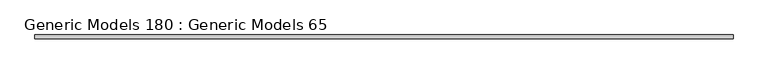
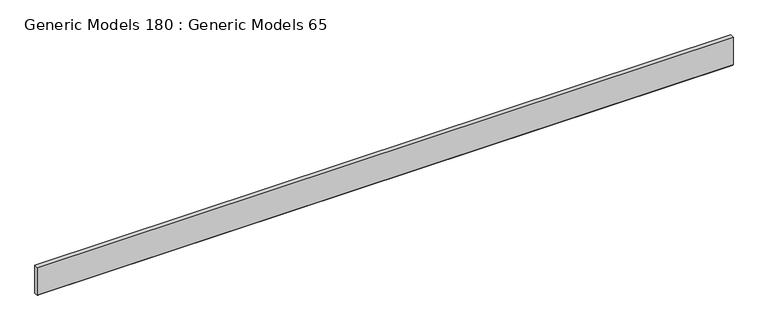
"""IFC4 building model written with IfcOpenShell, lengths in millimetres: proxy geometry, Generic Models 180 : Generic Models 65."""

from ifc_helpers import new_model, si_unit, frame, origin, place, context, project, spatial, polyline, outline, extrude, source, transform, mapped, element, save


def generic_models_180_generic_models_65_f377bfa4(model_context):
    return source(origin(), model_context, "Body", "SweptSolid", [
        extrude(outline(polyline([(528.6375, 1892.3), (547.6875, 1892.3), (547.6875, 1752.6), (529.828125, 1752.6), (528.6375, 1753.790625), (528.6375, 1892.3)])), frame((-251067.8875, 0.0, 0.0), z_axis=(1.0, 0.0, 0.0), x_axis=(0.0, 1.0, 0.0)), (0.0, 0.0, 1.0), 3289.3),
    ])


if __name__ == "__main__":
    model = new_model("IFC4")
    model_context = context("Model", 3, world=origin())
    ifc_project = project(units=[si_unit("LENGTHUNIT", "METRE", prefix="MILLI")], contexts=[model_context])
    site = spatial("IfcSite", under=ifc_project)
    building = spatial("IfcBuilding", under=site)
    placement = place(None, origin())
    generic_models_180_generic_models_65_shape = generic_models_180_generic_models_65_f377bfa4(model_context)
    element("IfcBuildingElementProxy", 1, Name="Generic Models 180 : Generic Models 65", ObjectType="Generic Models 180 : Generic Models 65", at=placement, inside=building, context=model_context, shape_type="MappedRepresentation", body=[
        mapped(generic_models_180_generic_models_65_shape, transform((0.0, 0.0, 0.0), x_axis=(1.0, 0.0, 0.0), y_axis=(0.0, 1.0, 0.0), z_axis=(0.0, 0.0, 1.0))),
    ])
    save(model, "model.ifc")

# Revit data of these elements
# Element 1 (IfcBuildingElementProxy, "Generic Models 180 : Generic Models 65")
#   Materials on its faces: "HORIZONTAL 1X6 CEDAR PLANKS W/ CLEAR WOOD SEALER"
# Materials
#   "HORIZONTAL 1X6 CEDAR PLANKS W/ CLEAR WOOD SEALER": class "Wood", colour RGB 234 198 147, transparency 0, Description = "Pinus Echinata", Cost = 0
